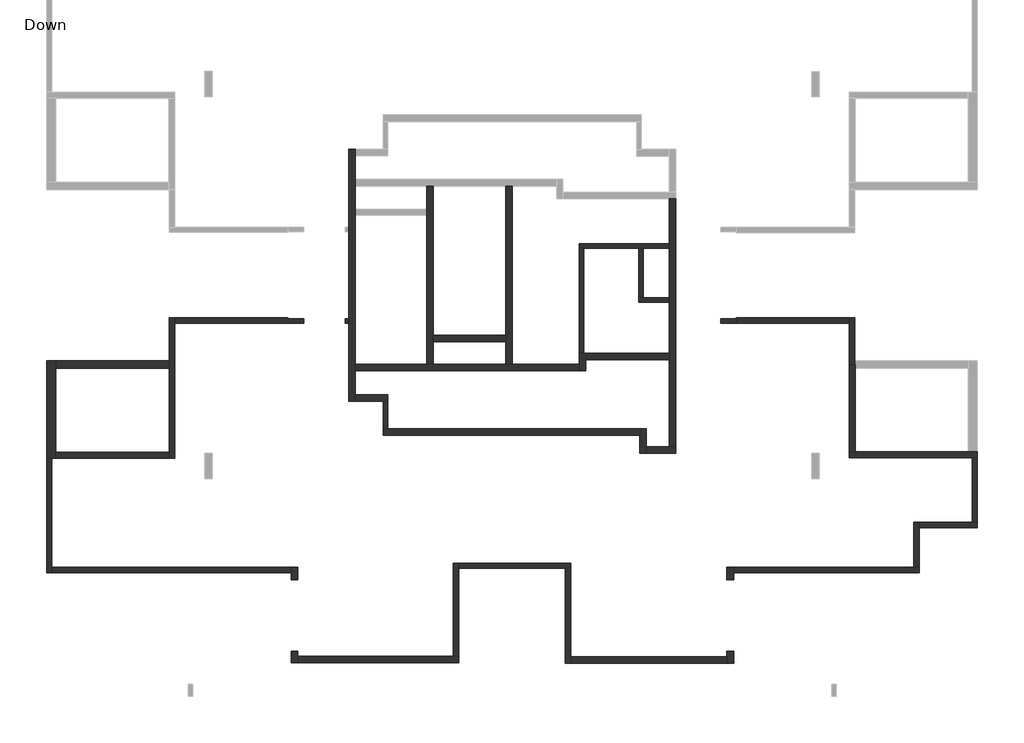
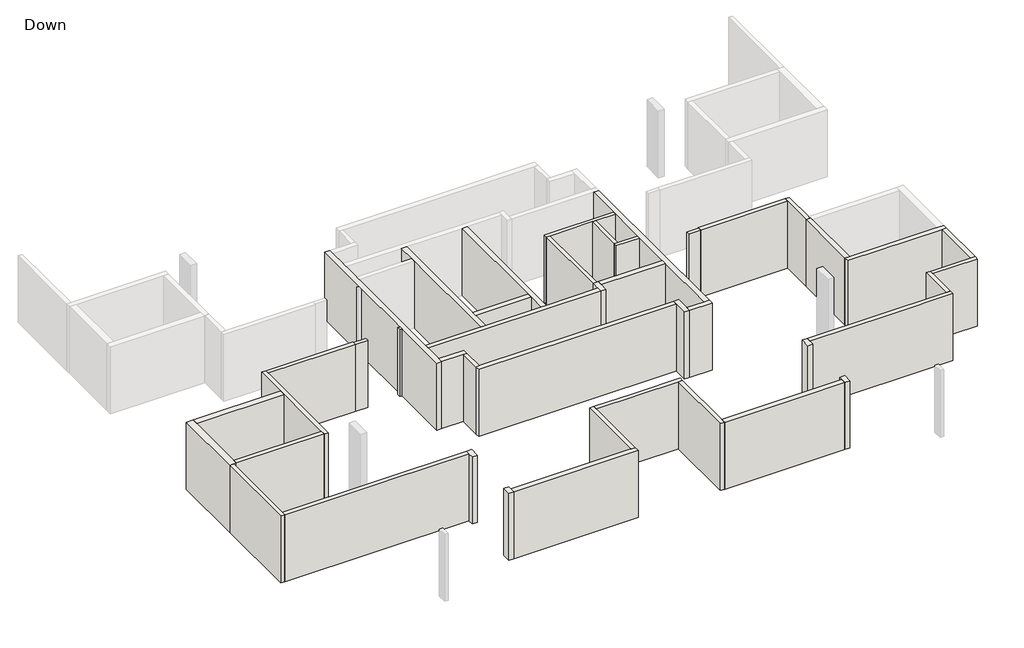
# One storey, part 1 of 2: 44 walls.
"""IFC4 building model written with IfcOpenShell, lengths in millimetres."""

from ifc_helpers import new_model, si_unit, origin, origin_with_axes, place, context, project, spatial, polyline, outline, extrude, faceted_brep, element, save

model = new_model("IFC4")

# Units and contexts
model_context = context("Model", 3, world=origin())
ifc_project = project(units=[si_unit("LENGTHUNIT", "METRE", prefix="MILLI")], contexts=[model_context])

# Site, building, storey
site = spatial("IfcSite", under=ifc_project)
building = spatial("IfcBuilding", under=site)
storey = spatial("IfcBuildingStorey", under=building, Name="Down", Elevation=0.0)

# Walls
placement = place(None, origin())
element("IfcWall", 1, ObjectType="15", at=placement, inside=storey, context=model_context, shape_type="Brep", body=[
    faceted_brep([(3307.48852, -2656.5516458, 0.0), (3822.84243, -2656.5516458, 0.0), (3822.84243, -2656.5516458, 3070.0), (3307.48852, -2656.5516458, 3070.0), (3307.48852, -2506.5516458, 0.0), (3307.48852, -2506.5516458, 3070.0), (3822.84243, -2506.5516458, 3070.0), (3822.84243, -2506.5516458, 2920.0), (3822.84243, -2506.5516458, 0.0), (3822.84243, -2656.2878227, 0.0), (3822.84243, -2656.2878227, 3070.0)], [[[0, 1, 2, 3]], [[4, 5, 6, 7, 8]], [[1, 0, 4, 8, 9]], [[2, 1, 9, 8, 7, 6, 10]], [[3, 2, 10, 6, 5]], [[0, 3, 5, 4]]]),
])
element("IfcWall", 2, ObjectType="15", at=placement, inside=storey, context=model_context, shape_type="Brep", body=[
    faceted_brep([(-11137.3486135, -2656.5516458, 0.0), (-10610.0280472, -2656.5516458, 0.0), (-10610.0280472, -2656.5516458, 2870.0), (-10610.0280472, -2656.5516458, 3070.0), (-11137.3486135, -2656.5516458, 3070.0), (-11137.3486135, -2656.5516458, 2870.0), (-11137.3486135, -2506.5516458, 0.0), (-11137.3486135, -2506.5516458, 2920.0), (-11137.3486135, -2506.5516458, 3070.0), (-10610.0280472, -2506.5516458, 3070.0), (-10610.0280472, -2506.5516458, 0.0), (-11137.3486135, -2656.2878227, 0.0), (-10610.0280472, -2655.7878227, 3070.0), (-11137.3486135, -2656.2878227, 3070.0)], [[[0, 1, 2, 3, 4, 5]], [[6, 7, 8, 9, 10]], [[1, 0, 11, 6, 10]], [[3, 2, 1, 10, 9, 12]], [[4, 3, 12, 9, 8, 13]], [[0, 5, 4, 13, 8, 7, 6, 11]]]),
])
element("IfcWall", 3, ObjectType="15", at=placement, inside=storey, context=model_context, shape_type="Brep", body=[
    faceted_brep([(-1415.2062248, -154.9895964, 0.0), (-1265.2062248, -154.9895964, 0.0), (579.9772808, -154.9895964, 0.0), (729.9772808, -154.9895964, 0.0), (1589.3005209, -154.9895964, 0.0), (1589.3005209, -154.9895964, 3070.0), (729.9772808, -154.9895964, 3070.0), (579.9772808, -154.9895964, 3070.0), (-1265.2062248, -154.9895964, 3070.0), (-1415.2062248, -154.9895964, 3070.0), (-1415.2062248, -4.9895964, 0.0), (-1415.2062248, -4.9895964, 2870.0), (-1415.2062248, -4.9895964, 3070.0), (1589.3005209, -4.9895964, 3070.0), (1589.3005209, -4.9895964, 2870.0), (1589.3005209, -4.9895964, 0.0)], [[[0, 1, 2, 3, 4, 5, 6, 7, 8, 9]], [[10, 11, 12, 13, 14, 15]], [[4, 3, 2, 1, 0, 10, 15]], [[9, 8, 7, 6, 5, 13, 12]], [[5, 4, 15, 14, 13]], [[0, 9, 12, 11, 10]]]),
])
element("IfcWall", 4, ObjectType="15", at=placement, inside=storey, context=model_context, shape_type="Brep", body=[
    faceted_brep([(1589.3005209, -1810.18983, 0.0), (729.9772808, -1810.18983, 0.0), (579.9772808, -1810.18983, 0.0), (579.9772808, -1810.18983, 3070.0), (729.9772808, -1810.18983, 3070.0), (1589.3005209, -1810.18983, 3070.0), (1589.3005209, -1960.18983, 0.0), (1589.3005209, -1960.18983, 3070.0), (579.9772808, -1960.18983, 3070.0), (579.9772808, -1960.18983, 0.0)], [[[0, 1, 2, 3, 4, 5]], [[6, 7, 8, 9]], [[2, 1, 0, 6, 9]], [[5, 4, 3, 8, 7]], [[0, 5, 7, 6]], [[3, 2, 9, 8]]]),
])
element("IfcWall", 5, ObjectType="15", at=placement, inside=storey, context=model_context, shape_type="SweptSolid", body=[
    extrude(outline(polyline([(579.9772808, -1810.18983), (579.9772808, -154.9895964), (729.9772808, -154.9895964), (729.9772808, -1810.18983), (579.9772808, -1810.18983)])), origin_with_axes(), (0.0, 0.0, 1.0), 3070.0),
])
element("IfcWall", 6, ObjectType="15", at=placement, inside=storey, context=model_context, shape_type="SweptSolid", body=[
    extrude(outline(polyline([(-1415.2062248, -3664.0679171), (-1415.2062248, -154.9895964), (-1265.2062248, -154.9895964), (-1265.2062248, -3664.0679171), (-1415.2062248, -3664.0679171)])), origin_with_axes(), (0.0, 0.0, 1.0), 3070.0),
])
element("IfcWall", 7, ObjectType="15", at=placement, inside=storey, context=model_context, shape_type="Brep", body=[
    faceted_brep([(-7960.7109614, -5263.3286489, 0.0), (-7960.7109614, -6190.6239212, 0.0), (-7960.7109614, -6190.6239212, 3070.0), (-7960.7109614, -5263.3286489, 3070.0), (-7960.7109614, -5263.3286489, 2870.0), (-7810.7109614, -5263.3286489, 0.0), (-7810.7109614, -5263.3286489, 3070.0), (-7810.7109614, -6190.6239212, 3070.0), (-7810.7109614, -6190.6239212, 2870.0), (-7810.7109614, -6190.6239212, 0.0)], [[[0, 1, 2, 3, 4]], [[5, 6, 7, 8, 9]], [[1, 0, 5, 9]], [[3, 2, 7, 6]], [[0, 4, 3, 6, 5]], [[2, 1, 9, 8, 7]]]),
])
element("IfcWall", 8, ObjectType="15", at=placement, inside=storey, context=model_context, shape_type="Brep", body=[
    faceted_brep([(-9219.5481077, -2656.5516458, 0.0), (-9111.0923752, -2656.5516458, 0.0), (-9111.0923752, -2656.5516458, 2870.0), (-9111.0923752, -2656.5516458, 3070.0), (-9219.5481077, -2656.5516458, 3070.0), (-9219.5481077, -2656.5516458, 2870.0), (-9219.5481077, -2506.5516458, 0.0), (-9219.5481077, -2506.5516458, 3070.0), (-9111.0923752, -2506.5516458, 3070.0), (-9111.0923752, -2506.5516458, 2920.0), (-9111.0923752, -2506.5516458, 0.0), (-9219.5481077, -2655.7878227, 3070.0)], [[[0, 1, 2, 3, 4, 5]], [[6, 7, 8, 9, 10]], [[1, 0, 6, 10]], [[4, 3, 8, 7, 11]], [[0, 5, 4, 11, 7, 6]], [[3, 2, 1, 10, 9, 8]]]),
])
element("IfcWall", 9, ObjectType="18", at=placement, inside=storey, context=model_context, shape_type="Brep", body=[
    faceted_brep([(-15093.3730612, -2476.2878227, 0.0), (-15093.3730612, -3916.1341463, 0.0), (-15093.3730612, -4166.1341463, 0.0), (-15093.3730612, -6966.8226087, 0.0), (-15093.3730612, -7166.8226087, 0.0), (-15093.3730612, -7166.8226087, 3070.0), (-15093.3730612, -6966.8226087, 3070.0), (-15093.3730612, -4166.1341463, 3070.0), (-15093.3730612, -3916.1341463, 3070.0), (-15093.3730612, -2476.2878227, 3070.0), (-14913.3730612, -2476.2878227, 0.0), (-14913.3730612, -2476.2878227, 3070.0), (-14913.3730612, -2656.2878227, 3070.0), (-14913.3730612, -7166.8226087, 3070.0), (-14913.3730612, -7166.8226087, 2870.0), (-14913.3730612, -7166.8226087, 0.0), (-14913.3730612, -2656.2878227, 0.0)], [[[0, 1, 2, 3, 4, 5, 6, 7, 8, 9]], [[10, 11, 12, 13, 14, 15, 16]], [[4, 3, 2, 1, 0, 10, 16, 15]], [[9, 8, 7, 6, 5, 13, 12, 11]], [[5, 4, 15, 14, 13]], [[0, 9, 11, 10]]]),
])
element("IfcWall", 10, ObjectType="18", at=placement, inside=storey, context=model_context, shape_type="Brep", body=[
    faceted_brep([(-19192.7470995, -7166.8226087, 0.0), (-19192.7470995, -10993.4504981, 0.0), (-19192.7470995, -10993.4504981, 3070.0), (-19192.7470995, -7166.8226087, 3070.0), (-19012.7470995, -7166.8226087, 0.0), (-19012.7470995, -7166.8226087, 2870.0), (-19012.7470995, -7166.8226087, 3070.0), (-19012.7470995, -10813.4504981, 3070.0), (-19012.7470995, -10993.4504981, 3070.0), (-19012.7470995, -10993.4504981, 0.0), (-19012.7470995, -10813.4504981, 0.0)], [[[0, 1, 2, 3]], [[4, 5, 6, 7, 8, 9, 10]], [[1, 0, 4, 10, 9]], [[3, 2, 8, 7, 6]], [[0, 3, 6, 5, 4]], [[2, 1, 9, 8]]]),
])
element("IfcWall", 11, ObjectType="18", at=placement, inside=storey, context=model_context, shape_type="Brep", body=[
    faceted_brep([(-19012.7470995, -10993.4504981, 0.0), (-11029.6404044, -10993.4504981, 0.0), (-11029.6404044, -10993.4504981, 2870.0), (-11029.6404044, -10993.4504981, 3070.0), (-14463.9862657, -10993.4504981, 3070.0), (-19012.7470995, -10993.4504981, 3070.0), (-19012.7470995, -10813.4504981, 0.0), (-19012.7470995, -10813.4504981, 2870.0), (-19012.7470995, -10813.4504981, 3070.0), (-11029.6404044, -10813.4504981, 3070.0), (-11029.6404044, -10813.4504981, 0.0)], [[[0, 1, 2, 3, 4, 5]], [[6, 7, 8, 9, 10]], [[1, 0, 6, 10]], [[5, 4, 3, 9, 8]], [[0, 5, 8, 7, 6]], [[3, 2, 1, 10, 9]]]),
])
element("IfcWall", 12, ObjectType="18", at=placement, inside=storey, context=model_context, shape_type="Brep", body=[
    faceted_brep([(-5611.3302453, -10669.5773003, 0.0), (-5611.3302453, -13772.0681688, 0.0), (-5611.3302453, -13772.0681688, 2870.0), (-5611.3302453, -13772.0681688, 3070.0), (-5611.3302453, -10669.5773003, 3070.0), (-5611.3302453, -10669.5773003, 2870.0), (-5431.3302453, -10669.5773003, 0.0), (-5431.3302453, -10669.5773003, 3070.0), (-5431.3302453, -10849.5773003, 3070.0), (-5431.3302453, -13772.0681688, 3070.0), (-5431.3302453, -13772.0681688, 0.0), (-5431.3302453, -10849.5773003, 0.0)], [[[0, 1, 2, 3, 4, 5]], [[6, 7, 8, 9, 10, 11]], [[1, 0, 6, 11, 10]], [[4, 3, 9, 8, 7]], [[3, 2, 1, 10, 9]], [[0, 5, 4, 7, 6]]]),
])
element("IfcWall", 13, ObjectType="18", at=placement, inside=storey, context=model_context, shape_type="Brep", body=[
    faceted_brep([(-5431.3302453, -10849.5773003, 0.0), (-1871.2080852, -10849.5773003, 0.0), (-1691.2080852, -10849.5773003, 0.0), (-1691.2080852, -10849.5773003, 3070.0), (-1871.2080852, -10849.5773003, 3070.0), (-5431.3302453, -10849.5773003, 3070.0), (-5431.3302453, -10669.5773003, 0.0), (-5431.3302453, -10669.5773003, 3070.0), (-3748.3678079, -10669.5773003, 3070.0), (-3553.3678079, -10669.5773003, 3070.0), (-1691.2080852, -10669.5773003, 3070.0), (-1691.2080852, -10669.5773003, 2870.0), (-1691.2080852, -10669.5773003, 0.0)], [[[0, 1, 2, 3, 4, 5]], [[6, 7, 8, 9, 10, 11, 12]], [[2, 1, 0, 6, 12]], [[5, 4, 3, 10, 9, 8, 7]], [[0, 5, 7, 6]], [[3, 2, 12, 11, 10]]]),
])
element("IfcWall", 14, ObjectType="18", at=placement, inside=storey, context=model_context, shape_type="Brep", body=[
    faceted_brep([(-1871.2080852, -10849.5773003, 0.0), (-1871.2080852, -14009.5773003, 0.0), (-1871.2080852, -14009.5773003, 3070.0), (-1871.2080852, -10849.5773003, 3070.0), (-1691.2080852, -10849.5773003, 0.0), (-1691.2080852, -10849.5773003, 3070.0), (-1691.2080852, -13789.5773003, 3070.0), (-1691.2080852, -14009.5773003, 3070.0), (-1691.2080852, -14009.5773003, 0.0), (-1691.2080852, -13789.5773003, 0.0)], [[[0, 1, 2, 3]], [[4, 5, 6, 7, 8, 9]], [[1, 0, 4, 9, 8]], [[3, 2, 7, 6, 5]], [[0, 3, 5, 4]], [[2, 1, 8, 7]]]),
])
element("IfcWall", 15, ObjectType="18", at=placement, inside=storey, context=model_context, shape_type="Brep", body=[
    faceted_brep([(9937.2529005, -10813.4467583, 0.0), (9757.2529005, -10813.4467583, 0.0), (3739.0676082, -10813.4467583, 0.0), (3739.0676082, -10813.4467583, 3070.0), (9757.2529005, -10813.4467583, 3070.0), (9937.2529005, -10813.4467583, 3070.0), (9937.2529005, -10993.4467583, 0.0), (9937.2529005, -10993.4467583, 3070.0), (7161.4479352, -10993.4467583, 3070.0), (3739.0676082, -10993.4467583, 3070.0), (3739.0676082, -10993.4467583, 2870.0), (3739.0676082, -10993.4467583, 0.0)], [[[0, 1, 2, 3, 4, 5]], [[6, 7, 8, 9, 10, 11]], [[2, 1, 0, 6, 11]], [[5, 4, 3, 9, 8, 7]], [[0, 5, 7, 6]], [[3, 2, 11, 10, 9]]]),
])
element("IfcWall", 16, ObjectType="18", at=placement, inside=storey, context=model_context, shape_type="Brep", body=[
    faceted_brep([(9757.2529005, -9313.7627402, 0.0), (9757.2529005, -10813.4467583, 0.0), (9757.2529005, -10813.4467583, 2870.0), (9757.2529005, -10813.4467583, 3070.0), (9757.2529005, -9313.7627402, 3070.0), (9757.2529005, -9313.7627402, 2870.0), (9937.2529005, -9313.7627402, 0.0), (9937.2529005, -9313.7627402, 3070.0), (9937.2529005, -9493.7627402, 3070.0), (9937.2529005, -10813.4467583, 3070.0), (9937.2529005, -10813.4467583, 0.0), (9937.2529005, -9493.7627402, 0.0)], [[[0, 1, 2, 3, 4, 5]], [[6, 7, 8, 9, 10, 11]], [[1, 0, 6, 11, 10]], [[4, 3, 9, 8, 7]], [[3, 2, 1, 10, 9]], [[0, 5, 4, 7, 6]]]),
])
element("IfcWall", 17, ObjectType="18", at=placement, inside=storey, context=model_context, shape_type="Brep", body=[
    faceted_brep([(9937.2529005, -9493.7627402, 0.0), (11878.5007748, -9493.7627402, 0.0), (11878.5007748, -9493.7627402, 3070.0), (9937.2529005, -9493.7627402, 3070.0), (9937.2529005, -9313.7627402, 0.0), (9937.2529005, -9313.7627402, 3070.0), (11698.5007748, -9313.7627402, 3070.0), (11878.5007748, -9313.7627402, 3070.0), (11878.5007748, -9313.7627402, 0.0), (11698.5007748, -9313.7627402, 0.0)], [[[0, 1, 2, 3]], [[4, 5, 6, 7, 8, 9]], [[1, 0, 4, 9, 8]], [[3, 2, 7, 6, 5]], [[0, 3, 5, 4]], [[2, 1, 8, 7]]]),
])
element("IfcWall", 18, ObjectType="18", at=placement, inside=storey, context=model_context, shape_type="Brep", body=[
    faceted_brep([(11878.5007748, -9313.7627402, 0.0), (11878.5007748, -7153.7627402, 0.0), (11878.5007748, -7153.7627402, 3070.0), (11878.5007748, -9313.7627402, 3070.0), (11698.5007748, -9313.7627402, 0.0), (11698.5007748, -9313.7627402, 2870.0), (11698.5007748, -9313.7627402, 3070.0), (11698.5007748, -7153.7627402, 3070.0), (11698.5007748, -7153.7627402, 2870.0), (11698.5007748, -7153.7627402, 0.0)], [[[0, 1, 2, 3]], [[4, 5, 6, 7, 8, 9]], [[1, 0, 4, 9]], [[3, 2, 7, 6]], [[0, 3, 6, 5, 4]], [[2, 1, 9, 8, 7]]]),
])
element("IfcWall", 19, ObjectType="18", at=placement, inside=storey, context=model_context, shape_type="Brep", body=[
    faceted_brep([(7780.4432059, -4041.1341463, 0.0), (7780.4432059, -3916.1341463, 0.0), (7780.4432059, -2476.2878227, 0.0), (7780.4432059, -2476.2878227, 3070.0), (7780.4432059, -3916.1341463, 3070.0), (7780.4432059, -4041.1341463, 3070.0), (7600.4432059, -4041.1341463, 0.0), (7600.4432059, -4041.1341463, 3070.0), (7600.4432059, -2656.5516458, 3070.0), (7600.4432059, -2656.2878227, 3070.0), (7600.4432059, -2476.2878227, 3070.0), (7600.4432059, -2476.2878227, 0.0), (7600.4432059, -2656.2878227, 0.0)], [[[0, 1, 2, 3, 4, 5]], [[6, 7, 8, 9, 10, 11, 12]], [[2, 1, 0, 6, 12, 11]], [[5, 4, 3, 10, 9, 8, 7]], [[0, 5, 7, 6]], [[3, 2, 11, 10]]]),
])
element("IfcWall", 20, ObjectType="18", at=placement, inside=storey, context=model_context, shape_type="Brep", body=[
    faceted_brep([(7600.4432059, -2476.2878227, 0.0), (3822.84243, -2476.2878227, 0.0), (3822.84243, -2476.2878227, 3070.0), (7600.4432059, -2476.2878227, 3070.0), (7600.4432059, -2656.2878227, 0.0), (7600.4432059, -2656.2878227, 3070.0), (3822.84243, -2656.2878227, 3070.0), (3822.84243, -2656.2878227, 0.0), (3822.84243, -2506.5516458, 0.0), (3822.84243, -2506.5516458, 3070.0)], [[[0, 1, 2, 3]], [[4, 5, 6, 7]], [[1, 0, 4, 7, 8]], [[2, 1, 8, 7, 6, 9]], [[3, 2, 9, 6, 5]], [[0, 3, 5, 4]]]),
])
element("IfcWall", 21, ObjectType="18", at=placement, inside=storey, context=model_context, shape_type="Brep", body=[
    faceted_brep([(-14913.3730612, -2656.2878227, 0.0), (-11137.3486135, -2656.2878227, 0.0), (-11137.3486135, -2656.2878227, 2870.0), (-11137.3486135, -2656.2878227, 3070.0), (-14913.3730612, -2656.2878227, 3070.0), (-14913.3730612, -2656.2878227, 2870.0), (-14913.3730612, -2476.2878227, 0.0), (-14913.3730612, -2476.2878227, 3070.0), (-11137.3486135, -2476.2878227, 3070.0), (-11137.3486135, -2476.2878227, 0.0), (-11137.3486135, -2506.5516458, 0.0), (-11137.3486135, -2506.5516458, 3070.0)], [[[0, 1, 2, 3, 4, 5]], [[6, 7, 8, 9]], [[1, 0, 6, 9, 10]], [[3, 2, 1, 10, 9, 8, 11]], [[4, 3, 11, 8, 7]], [[0, 5, 4, 7, 6]]]),
])
element("IfcWall", 22, ObjectType="20", at=placement, inside=storey, context=model_context, shape_type="Brep", body=[
    faceted_brep([(-15093.3730612, -6966.8226087, 0.0), (-18893.0716357, -6966.8226087, 0.0), (-18893.0716357, -6966.8226087, 2870.0), (-18893.0716357, -6966.8226087, 3070.0), (-15093.3730612, -6966.8226087, 3070.0), (-15093.3730612, -6966.8226087, 2870.0), (-15093.3730612, -7166.8226087, 0.0), (-15093.3730612, -7166.8226087, 3070.0), (-18893.0716357, -7166.8226087, 3070.0), (-18893.0716357, -7166.8226087, 0.0)], [[[0, 1, 2, 3, 4, 5]], [[6, 7, 8, 9]], [[1, 0, 6, 9]], [[4, 3, 8, 7]], [[3, 2, 1, 9, 8]], [[0, 5, 4, 7, 6]]]),
])
element("IfcWall", 23, ObjectType="20", at=placement, inside=storey, context=model_context, shape_type="Brep", body=[
    faceted_brep([(11879.3119283, -6953.7627402, 0.0), (11579.3119283, -6953.7627402, 0.0), (7800.4432059, -6953.7627402, 0.0), (7600.4432059, -6953.7627402, 0.0), (7600.4432059, -6953.7627402, 3070.0), (7800.4432059, -6953.7627402, 3070.0), (11579.3119283, -6953.7627402, 3070.0), (11879.3119283, -6953.7627402, 3070.0), (11879.3119283, -7153.7627402, 0.0), (11879.3119283, -7153.7627402, 3070.0), (11878.5007748, -7153.7627402, 3070.0), (11698.5007748, -7153.7627402, 3070.0), (7600.4432059, -7153.7627402, 3070.0), (7600.4432059, -7153.7627402, 2870.0), (7600.4432059, -7153.7627402, 0.0), (11698.5007748, -7153.7627402, 0.0), (11878.5007748, -7153.7627402, 0.0)], [[[0, 1, 2, 3, 4, 5, 6, 7]], [[8, 9, 10, 11, 12, 13, 14, 15, 16]], [[3, 2, 1, 0, 8, 16, 15, 14]], [[7, 6, 5, 4, 12, 11, 10, 9]], [[0, 7, 9, 8]], [[4, 3, 14, 13, 12]]]),
])
element("IfcWall", 24, ObjectType="20", at=placement, inside=storey, context=model_context, shape_type="Brep", body=[
    faceted_brep([(7800.4432059, -6953.7627402, 0.0), (7800.4432059, -4166.1341463, 0.0), (7800.4432059, -4041.1341463, 0.0), (7800.4432059, -4041.1341463, 3070.0), (7800.4432059, -4166.1341463, 3070.0), (7800.4432059, -6953.7627402, 3070.0), (7800.4432059, -6953.7627402, 2870.0), (7600.4432059, -6953.7627402, 0.0), (7600.4432059, -6953.7627402, 3070.0), (7600.4432059, -4041.1341463, 3070.0), (7600.4432059, -4041.1341463, 0.0), (7780.4432059, -4041.1341463, 0.0), (7780.4432059, -4041.1341463, 3070.0)], [[[0, 1, 2, 3, 4, 5, 6]], [[7, 8, 9, 10]], [[2, 1, 0, 7, 10, 11]], [[3, 2, 11, 10, 9, 12]], [[5, 4, 3, 12, 9, 8]], [[0, 6, 5, 8, 7]]]),
])
element("IfcWall", 25, ObjectType="22", at=placement, inside=storey, context=model_context, shape_type="Brep", body=[
    faceted_brep([(-10809.6404044, -13992.0681688, 0.0), (-5431.0686661, -13992.0681688, 0.0), (-5431.0686661, -13992.0681688, 3070.0), (-10809.6404044, -13992.0681688, 3070.0), (-10809.6404044, -13772.0681688, 0.0), (-10809.6404044, -13772.0681688, 2870.0), (-10809.6404044, -13772.0681688, 3070.0), (-5611.3302453, -13772.0681688, 3070.0), (-5431.3302453, -13772.0681688, 3070.0), (-5431.0686661, -13772.0681688, 3070.0), (-5431.0686661, -13772.0681688, 0.0), (-5431.3302453, -13772.0681688, 0.0), (-5611.3302453, -13772.0681688, 0.0)], [[[0, 1, 2, 3]], [[4, 5, 6, 7, 8, 9, 10, 11, 12]], [[1, 0, 4, 12, 11, 10]], [[2, 1, 10, 9]], [[3, 2, 9, 8, 7, 6]], [[0, 3, 6, 5, 4]]]),
])
element("IfcWall", 26, ObjectType="22", at=placement, inside=storey, context=model_context, shape_type="Brep", body=[
    faceted_brep([(3519.0676082, -13789.5773003, 0.0), (-1691.2080852, -13789.5773003, 0.0), (-1691.2080852, -13789.5773003, 2870.0), (-1691.2080852, -13789.5773003, 3070.0), (3519.0676082, -13789.5773003, 3070.0), (3519.0676082, -13789.5773003, 2870.0), (3519.0676082, -14009.5773003, 0.0), (3519.0676082, -14009.5773003, 3070.0), (-1691.2080852, -14009.5773003, 3070.0), (-1691.2080852, -14009.5773003, 0.0)], [[[0, 1, 2, 3, 4, 5]], [[6, 7, 8, 9]], [[1, 0, 6, 9]], [[4, 3, 8, 7]], [[3, 2, 1, 9, 8]], [[0, 5, 4, 7, 6]]]),
])
element("IfcWall", 27, ObjectType="22", at=placement, inside=storey, context=model_context, shape_type="Brep", body=[
    faceted_brep([(-8891.0923752, -5263.3286489, 0.0), (-8891.0923752, -5043.3286489, 0.0), (-8891.0923752, -4251.9774411, 0.0), (-8891.0923752, -4031.9774411, 0.0), (-8891.0923752, 942.6898033, 0.0), (-8891.0923752, 1142.6898033, 0.0), (-8891.0923752, 1914.3048342, 0.0), (-8891.0923752, 2134.3048342, 0.0), (-8891.0923752, 2921.8256682, 0.0), (-8891.0923752, 3141.8256682, 0.0), (-8891.0923752, 3141.8256682, 3070.0), (-8891.0923752, 2921.8256682, 3070.0), (-8891.0923752, 2134.3048342, 3070.0), (-8891.0923752, 1914.3048342, 3070.0), (-8891.0923752, 1142.6898033, 3070.0), (-8891.0923752, 942.6898033, 3070.0), (-8891.0923752, -4031.9774411, 3070.0), (-8891.0923752, -4251.9774411, 3070.0), (-8891.0923752, -5043.3286489, 3070.0), (-8891.0923752, -5263.3286489, 3070.0), (-9111.0923752, -5263.3286489, 0.0), (-9111.0923752, -5263.3286489, 2870.0), (-9111.0923752, -5263.3286489, 3070.0), (-9111.0923752, -2656.5516458, 3070.0), (-9111.0923752, -2506.5516458, 3070.0), (-9111.0923752, 396.2654793, 3070.0), (-9111.0923752, 546.2654793, 3070.0), (-9111.0923752, 3141.8256682, 3070.0), (-9111.0923752, 3141.8256682, 2870.0), (-9111.0923752, 3141.8256682, 0.0), (-9111.0923752, 546.2654793, 0.0), (-9111.0923752, 396.2654793, 0.0), (-9111.0923752, -2506.5516458, 0.0), (-9111.0923752, -2656.5516458, 0.0)], [[[0, 1, 2, 3, 4, 5, 6, 7, 8, 9, 10, 11, 12, 13, 14, 15, 16, 17, 18, 19]], [[20, 21, 22, 23, 24, 25, 26, 27, 28, 29, 30, 31, 32, 33]], [[9, 8, 7, 6, 5, 4, 3, 2, 1, 0, 20, 33, 32, 31, 30, 29]], [[19, 18, 17, 16, 15, 14, 13, 12, 11, 10, 27, 26, 25, 24, 23, 22]], [[10, 9, 29, 28, 27]], [[0, 19, 22, 21, 20]]]),
])
element("IfcWall", 28, ObjectType="22", at=placement, inside=storey, context=model_context, shape_type="Brep", body=[
    faceted_brep([(-7810.7109614, -5043.3286489, 0.0), (-8891.0923752, -5043.3286489, 0.0), (-8891.0923752, -5043.3286489, 2870.0), (-8891.0923752, -5043.3286489, 3070.0), (-7810.7109614, -5043.3286489, 3070.0), (-7810.7109614, -5043.3286489, 2870.0), (-7810.7109614, -5263.3286489, 0.0), (-7810.7109614, -5263.3286489, 3070.0), (-7960.7109614, -5263.3286489, 3070.0), (-8891.0923752, -5263.3286489, 3070.0), (-8891.0923752, -5263.3286489, 0.0), (-7960.7109614, -5263.3286489, 0.0)], [[[0, 1, 2, 3, 4, 5]], [[6, 7, 8, 9, 10, 11]], [[1, 0, 6, 11, 10]], [[4, 3, 9, 8, 7]], [[3, 2, 1, 10, 9]], [[0, 5, 4, 7, 6]]]),
])
element("IfcWall", 29, ObjectType="22", at=placement, inside=storey, context=model_context, shape_type="Brep", body=[
    faceted_brep([(-7960.7109614, -6410.6239212, 0.0), (610.3012935, -6410.6239212, 0.0), (610.3012935, -6410.6239212, 2870.0), (610.3012935, -6410.6239212, 3070.0), (-3553.3678079, -6410.6239212, 3070.0), (-3748.3678079, -6410.6239212, 3070.0), (-7960.7109614, -6410.6239212, 3070.0), (-7960.7109614, -6410.6239212, 2870.0), (-7960.7109614, -6190.6239212, 0.0), (-7960.7109614, -6190.6239212, 3070.0), (-7810.7109614, -6190.6239212, 3070.0), (610.3012935, -6190.6239212, 3070.0), (610.3012935, -6190.6239212, 0.0), (-7810.7109614, -6190.6239212, 0.0)], [[[0, 1, 2, 3, 4, 5, 6, 7]], [[8, 9, 10, 11, 12, 13]], [[1, 0, 8, 13, 12]], [[6, 5, 4, 3, 11, 10, 9]], [[0, 7, 6, 9, 8]], [[3, 2, 1, 12, 11]]]),
])
element("IfcWall", 30, ObjectType="22", at=placement, inside=storey, context=model_context, shape_type="Brep", body=[
    faceted_brep([(1809.3005209, -6790.4989795, 0.0), (1589.3005209, -6790.4989795, 0.0), (830.3012935, -6790.4989795, 0.0), (830.3012935, -6790.4989795, 2870.0), (830.3012935, -6790.4989795, 3070.0), (1589.3005209, -6790.4989795, 3070.0), (1809.3005209, -6790.4989795, 3070.0), (1809.3005209, -7010.4989795, 0.0), (1809.3005209, -7010.4989795, 2870.0), (1809.3005209, -7010.4989795, 3070.0), (830.3012935, -7010.4989795, 3070.0), (830.3012935, -7010.4989795, 0.0)], [[[0, 1, 2, 3, 4, 5, 6]], [[7, 8, 9, 10, 11]], [[2, 1, 0, 7, 11]], [[6, 5, 4, 10, 9]], [[4, 3, 2, 11, 10]], [[0, 6, 9, 8, 7]]]),
])
element("IfcWall", 31, ObjectType="22", at=placement, inside=storey, context=model_context, shape_type="Brep", body=[
    faceted_brep([(1809.3005209, -6790.4989795, 0.0), (1809.3005209, 1493.9448789, 0.0), (1809.3005209, 1493.9448789, 3070.0), (1809.3005209, 540.6860076, 3070.0), (1809.3005209, 390.6860076, 3070.0), (1809.3005209, -2506.5516458, 3070.0), (1809.3005209, -2656.5516458, 3070.0), (1809.3005209, -6790.4989795, 3070.0), (1589.3005209, -6790.4989795, 0.0), (1589.3005209, -6790.4989795, 2870.0), (1589.3005209, -6790.4989795, 3070.0), (1589.3005209, -3884.0679171, 3070.0), (1589.3005209, -3664.0679171, 3070.0), (1589.3005209, -1960.18983, 3070.0), (1589.3005209, -1810.18983, 3070.0), (1589.3005209, -154.9895964, 3070.0), (1589.3005209, -4.9895964, 3070.0), (1589.3005209, 1493.9448789, 3070.0), (1589.3005209, 1493.9448789, 2870.0), (1589.3005209, 1493.9448789, 0.0), (1589.3005209, -4.9895964, 0.0), (1589.3005209, -154.9895964, 0.0), (1589.3005209, -1810.18983, 0.0), (1589.3005209, -1960.18983, 0.0), (1589.3005209, -3664.0679171, 0.0), (1589.3005209, -3884.0679171, 0.0)], [[[0, 1, 2, 3, 4, 5, 6, 7]], [[8, 9, 10, 11, 12, 13, 14, 15, 16, 17, 18, 19, 20, 21, 22, 23, 24, 25]], [[1, 0, 8, 25, 24, 23, 22, 21, 20, 19]], [[7, 6, 5, 4, 3, 2, 17, 16, 15, 14, 13, 12, 11, 10]], [[2, 1, 19, 18, 17]], [[0, 7, 10, 9, 8]]]),
])
element("IfcWall", 32, ObjectType="22", at=placement, inside=storey, context=model_context, shape_type="Brep", body=[
    faceted_brep([(-1415.2062248, -4031.9774411, 0.0), (-3653.0437953, -4031.9774411, 0.0), (-3873.0437953, -4031.9774411, 0.0), (-6278.4263718, -4031.9774411, 0.0), (-6498.4263718, -4031.9774411, 0.0), (-8891.0923752, -4031.9774411, 0.0), (-8891.0923752, -4031.9774411, 2870.0), (-8891.0923752, -4031.9774411, 3070.0), (-6498.4263718, -4031.9774411, 3070.0), (-6278.4263718, -4031.9774411, 3070.0), (-3873.0437953, -4031.9774411, 3070.0), (-3653.0437953, -4031.9774411, 3070.0), (-1415.2062248, -4031.9774411, 3070.0), (-1415.2062248, -4031.9774411, 2870.0), (-1415.2062248, -4251.9774411, 0.0), (-1415.2062248, -4251.9774411, 3070.0), (-8891.0923752, -4251.9774411, 3070.0), (-8891.0923752, -4251.9774411, 2870.0), (-8891.0923752, -4251.9774411, 0.0)], [[[0, 1, 2, 3, 4, 5, 6, 7, 8, 9, 10, 11, 12, 13]], [[14, 15, 16, 17, 18]], [[5, 4, 3, 2, 1, 0, 14, 18]], [[12, 11, 10, 9, 8, 7, 16, 15]], [[7, 6, 5, 18, 17, 16]], [[0, 13, 12, 15, 14]]]),
])
element("IfcWall", 33, ObjectType="22", at=placement, inside=storey, context=model_context, shape_type="Brep", body=[
    faceted_brep([(-6278.4263718, -4031.9774411, 0.0), (-6278.4263718, -3284.1974214, 0.0), (-6278.4263718, -3064.1974214, 0.0), (-6278.4263718, 1914.3048342, 0.0), (-6278.4263718, 1914.3048342, 2870.0), (-6278.4263718, 1914.3048342, 3070.0), (-6278.4263718, -3064.1974214, 3070.0), (-6278.4263718, -3284.1974214, 3070.0), (-6278.4263718, -4031.9774411, 3070.0), (-6498.4263718, -4031.9774411, 0.0), (-6498.4263718, -4031.9774411, 2870.0), (-6498.4263718, -4031.9774411, 3070.0), (-6498.4263718, 942.6898033, 3070.0), (-6498.4263718, 1142.6898033, 3070.0), (-6498.4263718, 1914.3048342, 3070.0), (-6498.4263718, 1914.3048342, 0.0), (-6498.4263718, 1142.6898033, 0.0), (-6498.4263718, 942.6898033, 0.0)], [[[0, 1, 2, 3, 4, 5, 6, 7, 8]], [[9, 10, 11, 12, 13, 14, 15, 16, 17]], [[3, 2, 1, 0, 9, 17, 16, 15]], [[8, 7, 6, 5, 14, 13, 12, 11]], [[5, 4, 3, 15, 14]], [[0, 8, 11, 10, 9]]]),
])
element("IfcWall", 34, ObjectType="22", at=placement, inside=storey, context=model_context, shape_type="Brep", body=[
    faceted_brep([(-3653.0437953, -4031.9774411, 0.0), (-3653.0437953, 1914.3048342, 0.0), (-3653.0437953, 1914.3048342, 2870.0), (-3653.0437953, 1914.3048342, 3070.0), (-3653.0437953, -4031.9774411, 3070.0), (-3653.0437953, -4031.9774411, 2870.0), (-3873.0437953, -4031.9774411, 0.0), (-3873.0437953, -4031.9774411, 3070.0), (-3873.0437953, -3284.1974214, 3070.0), (-3873.0437953, -3064.1974214, 3070.0), (-3873.0437953, 1914.3048342, 3070.0), (-3873.0437953, 1914.3048342, 2870.0), (-3873.0437953, 1914.3048342, 0.0), (-3873.0437953, -3064.1974214, 0.0), (-3873.0437953, -3284.1974214, 0.0)], [[[0, 1, 2, 3, 4, 5]], [[6, 7, 8, 9, 10, 11, 12, 13, 14]], [[1, 0, 6, 14, 13, 12]], [[4, 3, 10, 9, 8, 7]], [[3, 2, 1, 12, 11, 10]], [[0, 5, 4, 7, 6]]]),
])
element("IfcWall", 35, ObjectType="22", at=placement, inside=storey, context=model_context, shape_type="Brep", body=[
    faceted_brep([(-3873.0437953, -3064.1974214, 0.0), (-6278.4263718, -3064.1974214, 0.0), (-6278.4263718, -3064.1974214, 2870.0), (-6278.4263718, -3064.1974214, 3070.0), (-3873.0437953, -3064.1974214, 3070.0), (-3873.0437953, -3064.1974214, 2870.0), (-3873.0437953, -3284.1974214, 0.0), (-3873.0437953, -3284.1974214, 3070.0), (-6278.4263718, -3284.1974214, 3070.0), (-6278.4263718, -3284.1974214, 0.0)], [[[0, 1, 2, 3, 4, 5]], [[6, 7, 8, 9]], [[1, 0, 6, 9]], [[4, 3, 8, 7]], [[0, 5, 4, 7, 6]], [[3, 2, 1, 9, 8]]]),
])
element("IfcWall", 36, ObjectType="22", at=placement, inside=storey, context=model_context, shape_type="Brep", body=[
    faceted_brep([(610.3012935, -6190.6239212, 0.0), (610.3012935, -6410.6239212, 0.0), (610.3012935, -7010.4989795, 0.0), (610.3012935, -7010.4989795, 2870.0), (610.3012935, -7010.4989795, 3070.0), (610.3012935, -6410.6239212, 3070.0), (610.3012935, -6190.6239212, 3070.0), (830.3012935, -6190.6239212, 0.0), (830.3012935, -6190.6239212, 2870.0), (830.3012935, -6190.6239212, 3070.0), (830.3012935, -6790.4989795, 3070.0), (830.3012935, -7010.4989795, 3070.0), (830.3012935, -7010.4989795, 0.0), (830.3012935, -6790.4989795, 0.0)], [[[0, 1, 2, 3, 4, 5, 6]], [[7, 8, 9, 10, 11, 12, 13]], [[2, 1, 0, 7, 13, 12]], [[6, 5, 4, 11, 10, 9]], [[0, 6, 9, 8, 7]], [[4, 3, 2, 12, 11]]]),
])
element("IfcWall", 37, ObjectType="22", at=placement, inside=storey, context=model_context, shape_type="Brep", body=[
    faceted_brep([(-1195.2062248, -3884.0679171, 0.0), (1589.3005209, -3884.0679171, 0.0), (1589.3005209, -3884.0679171, 2870.0), (1589.3005209, -3884.0679171, 3070.0), (-1195.2062248, -3884.0679171, 3070.0), (-1195.2062248, -3884.0679171, 2870.0), (-1195.2062248, -3664.0679171, 0.0), (-1195.2062248, -3664.0679171, 3070.0), (1589.3005209, -3664.0679171, 3070.0), (1589.3005209, -3664.0679171, 0.0)], [[[0, 1, 2, 3, 4, 5]], [[6, 7, 8, 9]], [[1, 0, 6, 9]], [[4, 3, 8, 7]], [[3, 2, 1, 9, 8]], [[0, 5, 4, 7, 6]]]),
])
element("IfcWall", 38, ObjectType="22", at=placement, inside=storey, context=model_context, shape_type="Brep", body=[
    faceted_brep([(-1415.2062248, -3664.0679171, 0.0), (-1415.2062248, -4031.9774411, 0.0), (-1415.2062248, -4251.9774411, 0.0), (-1415.2062248, -4251.9774411, 3070.0), (-1415.2062248, -4031.9774411, 3070.0), (-1415.2062248, -3664.0679171, 3070.0), (-1195.2062248, -3664.0679171, 0.0), (-1195.2062248, -3664.0679171, 3070.0), (-1195.2062248, -3884.0679171, 3070.0), (-1195.2062248, -4251.9774411, 3070.0), (-1195.2062248, -4251.9774411, 2870.0), (-1195.2062248, -4251.9774411, 0.0), (-1195.2062248, -3884.0679171, 0.0), (-1265.2062248, -3664.0679171, 0.0), (-1265.2062248, -3664.0679171, 3070.0)], [[[0, 1, 2, 3, 4, 5]], [[6, 7, 8, 9, 10, 11, 12]], [[2, 1, 0, 13, 6, 12, 11]], [[5, 4, 3, 9, 8, 7, 14]], [[3, 2, 11, 10, 9]], [[0, 5, 14, 7, 6, 13]]]),
])
element("IfcWall", 39, ObjectType="22", at=placement, inside=storey, context=model_context, shape_type="Brep", body=[
    faceted_brep([(-10809.6404044, -13992.0681688, 0.0), (-10809.6404044, -13772.0681688, 0.0), (-10809.6404044, -13620.3281962, 0.0), (-10809.6404044, -13620.3281962, 2420.0), (-10809.6404044, -13620.3281962, 3070.0), (-10809.6404044, -13772.0681688, 3070.0), (-10809.6404044, -13992.0681688, 3070.0), (-10809.6404044, -13992.0681688, 2870.0), (-11029.6404044, -13992.0681688, 0.0), (-11029.6404044, -13992.0681688, 2870.0), (-11029.6404044, -13992.0681688, 3070.0), (-11029.6404044, -13620.3281962, 3070.0), (-11029.6404044, -13620.3281962, 2420.0), (-11029.6404044, -13620.3281962, 0.0)], [[[0, 1, 2, 3, 4, 5, 6, 7]], [[8, 9, 10, 11, 12, 13]], [[2, 1, 0, 8, 13]], [[4, 3, 2, 13, 12, 11]], [[6, 5, 4, 11, 10]], [[0, 7, 6, 10, 9, 8]]]),
])
element("IfcWall", 40, ObjectType="22", at=placement, inside=storey, context=model_context, shape_type="Brep", body=[
    faceted_brep([(-11029.6404044, -10813.4504981, 0.0), (-11029.6404044, -10993.4504981, 0.0), (-11029.6404044, -11233.4504981, 0.0), (-11029.6404044, -11233.4504981, 2420.0), (-11029.6404044, -11233.4504981, 3070.0), (-11029.6404044, -10993.4504981, 3070.0), (-11029.6404044, -10813.4504981, 3070.0), (-10809.6404044, -10813.4504981, 0.0), (-10809.6404044, -10813.4504981, 2870.0), (-10809.6404044, -10813.4504981, 3070.0), (-10809.6404044, -11233.4504981, 3070.0), (-10809.6404044, -11233.4504981, 2420.0), (-10809.6404044, -11233.4504981, 0.0)], [[[0, 1, 2, 3, 4, 5, 6]], [[7, 8, 9, 10, 11, 12]], [[2, 1, 0, 7, 12]], [[4, 3, 2, 12, 11, 10]], [[6, 5, 4, 10, 9]], [[0, 6, 9, 8, 7]]]),
])
element("IfcWall", 41, ObjectType="22", at=placement, inside=storey, context=model_context, shape_type="Brep", body=[
    faceted_brep([(3739.0676082, -14009.5773003, 0.0), (3739.0676082, -13619.5773003, 0.0), (3739.0676082, -13619.5773003, 2420.0), (3739.0676082, -13619.5773003, 3070.0), (3739.0676082, -14009.5773003, 3070.0), (3739.0676082, -14009.5773003, 2870.0), (3519.0676082, -14009.5773003, 0.0), (3519.0676082, -14009.5773003, 2870.0), (3519.0676082, -14009.5773003, 3070.0), (3519.0676082, -13789.5773003, 3070.0), (3519.0676082, -13619.5773003, 3070.0), (3519.0676082, -13619.5773003, 2420.0), (3519.0676082, -13619.5773003, 0.0), (3519.0676082, -13789.5773003, 0.0)], [[[0, 1, 2, 3, 4, 5]], [[6, 7, 8, 9, 10, 11, 12, 13]], [[1, 0, 6, 13, 12]], [[3, 2, 1, 12, 11, 10]], [[4, 3, 10, 9, 8]], [[0, 5, 4, 8, 7, 6]]]),
])
element("IfcWall", 42, ObjectType="22", at=placement, inside=storey, context=model_context, shape_type="Brep", body=[
    faceted_brep([(3519.0676082, -10813.4467583, 0.0), (3519.0676082, -11233.4467583, 0.0), (3519.0676082, -11233.4467583, 2420.0), (3519.0676082, -11233.4467583, 3070.0), (3519.0676082, -10813.4467583, 3070.0), (3519.0676082, -10813.4467583, 2870.0), (3739.0676082, -10813.4467583, 0.0), (3739.0676082, -10813.4467583, 3070.0), (3739.0676082, -10993.4467583, 3070.0), (3739.0676082, -11233.4467583, 3070.0), (3739.0676082, -11233.4467583, 2420.0), (3739.0676082, -11233.4467583, 0.0), (3739.0676082, -10993.4467583, 0.0)], [[[0, 1, 2, 3, 4, 5]], [[6, 7, 8, 9, 10, 11, 12]], [[1, 0, 6, 12, 11]], [[3, 2, 1, 11, 10, 9]], [[4, 3, 9, 8, 7]], [[0, 5, 4, 7, 6]]]),
])
element("IfcWall", 43, ObjectType="25", at=placement, inside=storey, context=model_context, shape_type="Brep", body=[
    faceted_brep([(-15093.3730612, -3916.1341463, 0.0), (-18893.0716357, -3916.1341463, 0.0), (-18893.0716357, -3916.1341463, 3070.0), (-15093.3730612, -3916.1341463, 3070.0), (-15093.3730612, -4166.1341463, 0.0), (-15093.3730612, -4166.1341463, 2870.0), (-15093.3730612, -4166.1341463, 3070.0), (-18893.0716357, -4166.1341463, 3070.0), (-18893.0716357, -4166.1341463, 2870.0), (-18893.0716357, -4166.1341463, 0.0)], [[[0, 1, 2, 3]], [[4, 5, 6, 7, 8, 9]], [[1, 0, 4, 9]], [[3, 2, 7, 6]], [[2, 1, 9, 8, 7]], [[0, 3, 6, 5, 4]]]),
])
element("IfcWall", 44, ObjectType="30", at=placement, inside=storey, context=model_context, shape_type="Brep", body=[
    faceted_brep([(-19193.0716357, -3916.1341463, 0.0), (-19193.0716357, -7166.8226087, 0.0), (-19193.0716357, -7166.8226087, 3070.0), (-19193.0716357, -3916.1341463, 3070.0), (-18893.0716357, -3916.1341463, 0.0), (-18893.0716357, -3916.1341463, 3070.0), (-18893.0716357, -4166.1341463, 3070.0), (-18893.0716357, -6966.8226087, 3070.0), (-18893.0716357, -7166.8226087, 3070.0), (-18893.0716357, -7166.8226087, 0.0), (-18893.0716357, -6966.8226087, 0.0), (-18893.0716357, -4166.1341463, 0.0), (-19012.7470995, -7166.8226087, 0.0), (-19192.7470995, -7166.8226087, 0.0), (-19192.7470995, -7166.8226087, 3070.0), (-19012.7470995, -7166.8226087, 3070.0)], [[[0, 1, 2, 3]], [[4, 5, 6, 7, 8, 9, 10, 11]], [[1, 0, 4, 11, 10, 9, 12, 13]], [[3, 2, 14, 15, 8, 7, 6, 5]], [[0, 3, 5, 4]], [[2, 1, 13, 12, 9, 8, 15, 14]]]),
])

save(model, "model.ifc")

# Revit data of these elements
# Project information
#   Project Issue Date = "Issue Date"
#   Project Status = "Project Status"
#   Client Name = "לקוח"
#   Project Address = "Enter address here"
#   Project Name = "Project 001"
#   Project Number = "מספר פרויקט"
# Type "15"
#   Layers, outside or top first: 15 cm "Concrete" (function 1)
# Type "18"
#   Layers, outside or top first: 18 cm "Concrete" (function 1)
# Type "20"
#   Layers, outside or top first: 20 cm "Concrete" (function 1)
# Type "22"
#   Layers, outside or top first: 22 cm "Concrete" (function 1)
# Type "25"
#   Layers, outside or top first: 25 cm "Concrete" (function 1)
# Type "30"
#   Layers, outside or top first: 30 cm "Concrete" (function 1)
# Element 1 (IfcWall, "15")
#   Comments = ""
#   Mark = "W72"
#   SOFiSTiK_EdgeZones = "W72"
#   SOFiSTiK_AMG_Comments = ""
#   Top Offset = 0 cm
#   Base Offset = 0 cm
#   wall height = 307 cm
#   SOFiSTiK_AMG_Scheduled = yes
#   SOFiSTiK_AMG_Adjusted = yes
#   Phase Created = New Construction
#   Base Constraint = Down
#   Top Constraint = Typical Floor
#   Materials on its faces: "Concrete"
# Element 2 (IfcWall, "15")
#   Comments = ""
#   Mark = "W73"
#   SOFiSTiK_EdgeZones = "W73"
#   SOFiSTiK_AMG_Comments = ""
#   Top Offset = 0 cm
#   Base Offset = 0 cm
#   wall height = 307 cm
#   SOFiSTiK_AMG_Scheduled = yes
#   SOFiSTiK_AMG_Adjusted = yes
#   Phase Created = New Construction
#   Base Constraint = Down
#   Top Constraint = Typical Floor
#   Materials on its faces: "Concrete"
# Element 3 (IfcWall, "15")
#   Comments = ""
#   Mark = "W79"
#   SOFiSTiK_EdgeZones = "W79"
#   SOFiSTiK_AMG_Comments = ""
#   Top Offset = 0 cm
#   Base Offset = 0 cm
#   wall height = 307 cm
#   SOFiSTiK_AMG_Scheduled = yes
#   SOFiSTiK_AMG_Adjusted = yes
#   Phase Created = New Construction
#   Base Constraint = Down
#   Top Constraint = Typical Floor
#   Materials on its faces: "Concrete"
# Element 4 (IfcWall, "15")
#   Comments = ""
#   Mark = "W80"
#   SOFiSTiK_EdgeZones = "W80"
#   SOFiSTiK_AMG_Comments = ""
#   Top Offset = 0 cm
#   Base Offset = 0 cm
#   wall height = 307 cm
#   SOFiSTiK_AMG_Scheduled = yes
#   SOFiSTiK_AMG_Adjusted = yes
#   Phase Created = New Construction
#   Base Constraint = Down
#   Top Constraint = Typical Floor
#   Materials on its faces: "Concrete"
# Element 5 (IfcWall, "15")
#   Comments = ""
#   Mark = "W81"
#   SOFiSTiK_EdgeZones = "W81"
#   SOFiSTiK_AMG_Comments = ""
#   Top Offset = 0 cm
#   Base Offset = 0 cm
#   wall height = 307 cm
#   SOFiSTiK_AMG_Scheduled = yes
#   SOFiSTiK_AMG_Adjusted = yes
#   Phase Created = New Construction
#   Base Constraint = Down
#   Top Constraint = Typical Floor
#   Materials on its faces: "Concrete"
# Element 6 (IfcWall, "15")
#   Comments = ""
#   Mark = "W82"
#   SOFiSTiK_EdgeZones = "W82"
#   SOFiSTiK_AMG_Comments = ""
#   Top Offset = 0 cm
#   Base Offset = 0 cm
#   wall height = 307 cm
#   SOFiSTiK_AMG_Scheduled = yes
#   SOFiSTiK_AMG_Adjusted = yes
#   Phase Created = New Construction
#   Base Constraint = Down
#   Top Constraint = Typical Floor
#   Materials on its faces: "Concrete"
# Element 7 (IfcWall, "15")
#   Comments = ""
#   Mark = "W83"
#   SOFiSTiK_EdgeZones = "W83"
#   SOFiSTiK_AMG_Comments = ""
#   Top Offset = 0 cm
#   Base Offset = 0 cm
#   wall height = 307 cm
#   SOFiSTiK_AMG_Scheduled = yes
#   SOFiSTiK_AMG_Adjusted = yes
#   Phase Created = New Construction
#   Base Constraint = Down
#   Top Constraint = Typical Floor
#   Materials on its faces: "Concrete"
# Element 8 (IfcWall, "15")
#   Comments = ""
#   Mark = "W84"
#   SOFiSTiK_EdgeZones = "W84"
#   SOFiSTiK_AMG_Comments = "Too Short /"
#   Top Offset = 0 cm
#   Base Offset = 0 cm
#   wall height = 307 cm
#   SOFiSTiK_AMG_Scheduled = yes
#   SOFiSTiK_AMG_Adjusted = yes
#   Phase Created = New Construction
#   Base Constraint = Down
#   Top Constraint = Typical Floor
#   Materials on its faces: "Concrete"
# Element 9 (IfcWall, "18")
#   Comments = ""
#   Mark = "W5"
#   SOFiSTiK_EdgeZones = "W5"
#   SOFiSTiK_AMG_Comments = ""
#   Top Offset = 0 cm
#   Base Offset = 0 cm
#   wall height = 307 cm
#   SOFiSTiK_AMG_Scheduled = yes
#   SOFiSTiK_AMG_Adjusted = yes
#   Phase Created = New Construction
#   Base Constraint = Down
#   Top Constraint = Typical Floor
#   Materials on its faces: "Concrete"
# Element 10 (IfcWall, "18")
#   Comments = ""
#   Mark = "W6"
#   SOFiSTiK_EdgeZones = "W6"
#   SOFiSTiK_AMG_Comments = ""
#   Top Offset = 0 cm
#   Base Offset = 0 cm
#   wall height = 307 cm
#   SOFiSTiK_AMG_Scheduled = yes
#   SOFiSTiK_AMG_Adjusted = yes
#   Phase Created = New Construction
#   Base Constraint = Down
#   Top Constraint = Typical Floor
#   Materials on its faces: "Concrete"
# Element 11 (IfcWall, "18")
#   Comments = ""
#   Mark = "W7"
#   SOFiSTiK_EdgeZones = "W7"
#   SOFiSTiK_AMG_Comments = ""
#   Top Offset = 0 cm
#   Base Offset = 0 cm
#   wall height = 307 cm
#   SOFiSTiK_AMG_Scheduled = yes
#   SOFiSTiK_AMG_Adjusted = yes
#   Phase Created = New Construction
#   Base Constraint = Down
#   Top Constraint = Typical Floor
#   Materials on its faces: "Concrete"
# Element 12 (IfcWall, "18")
#   Comments = ""
#   Mark = "W8"
#   SOFiSTiK_EdgeZones = "W8"
#   SOFiSTiK_AMG_Comments = ""
#   Top Offset = 0 cm
#   Base Offset = 0 cm
#   wall height = 307 cm
#   SOFiSTiK_AMG_Scheduled = yes
#   SOFiSTiK_AMG_Adjusted = yes
#   Phase Created = New Construction
#   Base Constraint = Down
#   Top Constraint = Typical Floor
#   Materials on its faces: "Concrete"
# Element 13 (IfcWall, "18")
#   Comments = ""
#   Mark = "W9"
#   SOFiSTiK_EdgeZones = "W9"
#   SOFiSTiK_AMG_Comments = ""
#   Top Offset = 0 cm
#   Base Offset = 0 cm
#   wall height = 307 cm
#   SOFiSTiK_AMG_Scheduled = yes
#   SOFiSTiK_AMG_Adjusted = yes
#   Phase Created = New Construction
#   Base Constraint = Down
#   Top Constraint = Typical Floor
#   Materials on its faces: "Concrete"
# Element 14 (IfcWall, "18")
#   Comments = ""
#   Mark = "W10"
#   SOFiSTiK_EdgeZones = "W10"
#   SOFiSTiK_AMG_Comments = ""
#   Top Offset = 0 cm
#   Base Offset = 0 cm
#   wall height = 307 cm
#   SOFiSTiK_AMG_Scheduled = yes
#   SOFiSTiK_AMG_Adjusted = yes
#   Phase Created = New Construction
#   Base Constraint = Down
#   Top Constraint = Typical Floor
#   Materials on its faces: "Concrete"
# Element 15 (IfcWall, "18")
#   Comments = ""
#   Mark = "W11"
#   SOFiSTiK_EdgeZones = "W11"
#   SOFiSTiK_AMG_Comments = ""
#   Top Offset = 0 cm
#   Base Offset = 0 cm
#   wall height = 307 cm
#   SOFiSTiK_AMG_Scheduled = yes
#   SOFiSTiK_AMG_Adjusted = yes
#   Phase Created = New Construction
#   Base Constraint = Down
#   Top Constraint = Typical Floor
#   Materials on its faces: "Concrete"
# Element 16 (IfcWall, "18")
#   Comments = ""
#   Mark = "W12"
#   SOFiSTiK_EdgeZones = "W12"
#   SOFiSTiK_AMG_Comments = ""
#   Top Offset = 0 cm
#   Base Offset = 0 cm
#   wall height = 307 cm
#   SOFiSTiK_AMG_Scheduled = yes
#   SOFiSTiK_AMG_Adjusted = yes
#   Phase Created = New Construction
#   Base Constraint = Down
#   Top Constraint = Typical Floor
#   Materials on its faces: "Concrete"
# Element 17 (IfcWall, "18")
#   Comments = ""
#   Mark = "W13"
#   SOFiSTiK_EdgeZones = "W13"
#   SOFiSTiK_AMG_Comments = ""
#   Top Offset = 0 cm
#   Base Offset = 0 cm
#   wall height = 307 cm
#   SOFiSTiK_AMG_Scheduled = yes
#   SOFiSTiK_AMG_Adjusted = yes
#   Phase Created = New Construction
#   Base Constraint = Down
#   Top Constraint = Typical Floor
#   Materials on its faces: "Concrete"
# Element 18 (IfcWall, "18")
#   Comments = ""
#   Mark = "W14"
#   SOFiSTiK_EdgeZones = "W14"
#   SOFiSTiK_AMG_Comments = ""
#   Top Offset = 0 cm
#   Base Offset = 0 cm
#   wall height = 307 cm
#   SOFiSTiK_AMG_Scheduled = yes
#   SOFiSTiK_AMG_Adjusted = yes
#   Phase Created = New Construction
#   Base Constraint = Down
#   Top Constraint = Typical Floor
#   Materials on its faces: "Concrete"
# Element 19 (IfcWall, "18")
#   Comments = ""
#   Mark = "W15"
#   SOFiSTiK_EdgeZones = "W15"
#   SOFiSTiK_AMG_Comments = ""
#   Top Offset = 0 cm
#   Base Offset = 0 cm
#   wall height = 307 cm
#   SOFiSTiK_AMG_Scheduled = yes
#   SOFiSTiK_AMG_Adjusted = yes
#   Phase Created = New Construction
#   Base Constraint = Down
#   Top Constraint = Typical Floor
#   Materials on its faces: "Concrete"
# Element 20 (IfcWall, "18")
#   Comments = ""
#   Mark = "W16"
#   SOFiSTiK_EdgeZones = "W16"
#   SOFiSTiK_AMG_Comments = ""
#   Top Offset = 0 cm
#   Base Offset = 0 cm
#   wall height = 307 cm
#   SOFiSTiK_AMG_Scheduled = yes
#   SOFiSTiK_AMG_Adjusted = yes
#   Phase Created = New Construction
#   Base Constraint = Down
#   Top Constraint = Typical Floor
#   Materials on its faces: "Concrete"
# Element 21 (IfcWall, "18")
#   Comments = ""
#   Mark = "W17"
#   SOFiSTiK_EdgeZones = "W17"
#   SOFiSTiK_AMG_Comments = ""
#   Top Offset = 0 cm
#   Base Offset = 0 cm
#   wall height = 307 cm
#   SOFiSTiK_AMG_Scheduled = yes
#   SOFiSTiK_AMG_Adjusted = yes
#   Phase Created = New Construction
#   Base Constraint = Down
#   Top Constraint = Typical Floor
#   Materials on its faces: "Concrete"
# Element 22 (IfcWall, "20")
#   Comments = ""
#   Mark = "W33"
#   SOFiSTiK_EdgeZones = "W33"
#   SOFiSTiK_AMG_Comments = ""
#   Top Offset = 0 cm
#   Base Offset = 0 cm
#   wall height = 307 cm
#   SOFiSTiK_AMG_Scheduled = yes
#   SOFiSTiK_AMG_Adjusted = yes
#   Phase Created = New Construction
#   Base Constraint = Down
#   Top Constraint = Typical Floor
#   Materials on its faces: "Concrete"
# Element 23 (IfcWall, "20")
#   Comments = ""
#   Mark = "W34"
#   SOFiSTiK_EdgeZones = "W34"
#   SOFiSTiK_AMG_Comments = ""
#   Top Offset = 0 cm
#   Base Offset = 0 cm
#   wall height = 307 cm
#   SOFiSTiK_AMG_Scheduled = yes
#   SOFiSTiK_AMG_Adjusted = yes
#   Phase Created = New Construction
#   Base Constraint = Down
#   Top Constraint = Typical Floor
#   Materials on its faces: "Concrete"
# Element 24 (IfcWall, "20")
#   Comments = ""
#   Mark = "W35"
#   SOFiSTiK_EdgeZones = "W35"
#   SOFiSTiK_AMG_Comments = ""
#   Top Offset = 0 cm
#   Base Offset = 0 cm
#   wall height = 307 cm
#   SOFiSTiK_AMG_Scheduled = yes
#   SOFiSTiK_AMG_Adjusted = yes
#   Phase Created = New Construction
#   Base Constraint = Down
#   Top Constraint = Typical Floor
#   Materials on its faces: "Concrete"
# Element 25 (IfcWall, "22")
#   Comments = ""
#   Mark = "W42"
#   SOFiSTiK_EdgeZones = "W42"
#   SOFiSTiK_AMG_Comments = ""
#   Top Offset = 0 cm
#   Base Offset = 0 cm
#   wall height = 307 cm
#   SOFiSTiK_AMG_Scheduled = yes
#   SOFiSTiK_AMG_Adjusted = yes
#   Phase Created = New Construction
#   Base Constraint = Down
#   Top Constraint = Typical Floor
#   Materials on its faces: "Concrete"
# Element 26 (IfcWall, "22")
#   Comments = ""
#   Mark = "W43"
#   SOFiSTiK_EdgeZones = "W43"
#   SOFiSTiK_AMG_Comments = ""
#   Top Offset = 0 cm
#   Base Offset = 0 cm
#   wall height = 307 cm
#   SOFiSTiK_AMG_Scheduled = yes
#   SOFiSTiK_AMG_Adjusted = yes
#   Phase Created = New Construction
#   Base Constraint = Down
#   Top Constraint = Typical Floor
#   Materials on its faces: "Concrete"
# Element 27 (IfcWall, "22")
#   Comments = ""
#   Mark = "W44"
#   SOFiSTiK_EdgeZones = "W44"
#   SOFiSTiK_AMG_Comments = ""
#   Top Offset = 0 cm
#   Base Offset = 0 cm
#   wall height = 307 cm
#   SOFiSTiK_AMG_Scheduled = yes
#   SOFiSTiK_AMG_Adjusted = yes
#   Phase Created = New Construction
#   Base Constraint = Down
#   Top Constraint = Typical Floor
#   Materials on its faces: "Concrete"
# Element 28 (IfcWall, "22")
#   Comments = ""
#   Mark = "W53"
#   SOFiSTiK_EdgeZones = "W53"
#   SOFiSTiK_AMG_Comments = ""
#   Top Offset = 0 cm
#   Base Offset = 0 cm
#   wall height = 307 cm
#   SOFiSTiK_AMG_Scheduled = yes
#   SOFiSTiK_AMG_Adjusted = yes
#   Phase Created = New Construction
#   Base Constraint = Down
#   Top Constraint = Typical Floor
#   Materials on its faces: "Concrete"
# Element 29 (IfcWall, "22")
#   Comments = ""
#   Mark = "W54"
#   SOFiSTiK_EdgeZones = "W54"
#   SOFiSTiK_AMG_Comments = ""
#   Top Offset = 0 cm
#   Base Offset = 0 cm
#   wall height = 307 cm
#   SOFiSTiK_AMG_Scheduled = yes
#   SOFiSTiK_AMG_Adjusted = yes
#   Phase Created = New Construction
#   Base Constraint = Down
#   Top Constraint = Typical Floor
#   Materials on its faces: "Concrete"
# Element 30 (IfcWall, "22")
#   Comments = ""
#   Mark = "W55"
#   SOFiSTiK_EdgeZones = "W55"
#   SOFiSTiK_AMG_Comments = ""
#   Top Offset = 0 cm
#   Base Offset = 0 cm
#   wall height = 307 cm
#   SOFiSTiK_AMG_Scheduled = yes
#   SOFiSTiK_AMG_Adjusted = yes
#   Phase Created = New Construction
#   Base Constraint = Down
#   Top Constraint = Typical Floor
#   Materials on its faces: "Concrete"
# Element 31 (IfcWall, "22")
#   Comments = ""
#   Mark = "W56"
#   SOFiSTiK_EdgeZones = "W56"
#   SOFiSTiK_AMG_Comments = ""
#   Top Offset = 0 cm
#   Base Offset = 0 cm
#   wall height = 307 cm
#   SOFiSTiK_AMG_Scheduled = yes
#   SOFiSTiK_AMG_Adjusted = yes
#   Phase Created = New Construction
#   Base Constraint = Down
#   Top Constraint = Typical Floor
#   Materials on its faces: "Concrete"
# Element 32 (IfcWall, "22")
#   Comments = ""
#   Mark = "W57"
#   SOFiSTiK_EdgeZones = "W57"
#   SOFiSTiK_AMG_Comments = ""
#   Top Offset = 0 cm
#   Base Offset = 0 cm
#   wall height = 307 cm
#   SOFiSTiK_AMG_Scheduled = yes
#   SOFiSTiK_AMG_Adjusted = yes
#   Phase Created = New Construction
#   Base Constraint = Down
#   Top Constraint = Typical Floor
#   Materials on its faces: "Concrete"
# Element 33 (IfcWall, "22")
#   Comments = ""
#   Mark = "W58"
#   SOFiSTiK_EdgeZones = "W58"
#   SOFiSTiK_AMG_Comments = ""
#   Top Offset = 0 cm
#   Base Offset = 0 cm
#   wall height = 307 cm
#   SOFiSTiK_AMG_Scheduled = yes
#   SOFiSTiK_AMG_Adjusted = yes
#   Phase Created = New Construction
#   Base Constraint = Down
#   Top Constraint = Typical Floor
#   Materials on its faces: "Concrete"
# Element 34 (IfcWall, "22")
#   Comments = ""
#   Mark = "W59"
#   SOFiSTiK_EdgeZones = "W59"
#   SOFiSTiK_AMG_Comments = ""
#   Top Offset = 0 cm
#   Base Offset = 0 cm
#   wall height = 307 cm
#   SOFiSTiK_AMG_Scheduled = yes
#   SOFiSTiK_AMG_Adjusted = yes
#   Phase Created = New Construction
#   Base Constraint = Down
#   Top Constraint = Typical Floor
#   Materials on its faces: "Concrete"
# Element 35 (IfcWall, "22")
#   Comments = ""
#   Mark = "W60"
#   SOFiSTiK_EdgeZones = "W60"
#   SOFiSTiK_AMG_Comments = ""
#   Top Offset = 0 cm
#   Base Offset = 0 cm
#   wall height = 307 cm
#   SOFiSTiK_AMG_Scheduled = yes
#   SOFiSTiK_AMG_Adjusted = yes
#   Phase Created = New Construction
#   Base Constraint = Down
#   Top Constraint = Typical Floor
#   Materials on its faces: "Concrete"
# Element 36 (IfcWall, "22")
#   Comments = ""
#   Mark = "W61"
#   SOFiSTiK_EdgeZones = "W61"
#   SOFiSTiK_AMG_Comments = ""
#   Top Offset = 0 cm
#   Base Offset = 0 cm
#   wall height = 307 cm
#   SOFiSTiK_AMG_Scheduled = yes
#   SOFiSTiK_AMG_Adjusted = yes
#   Phase Created = New Construction
#   Base Constraint = Down
#   Top Constraint = Typical Floor
#   Materials on its faces: "Concrete"
# Element 37 (IfcWall, "22")
#   Comments = ""
#   Mark = "W62"
#   SOFiSTiK_EdgeZones = "W62"
#   SOFiSTiK_AMG_Comments = ""
#   Top Offset = 0 cm
#   Base Offset = 0 cm
#   wall height = 307 cm
#   SOFiSTiK_AMG_Scheduled = yes
#   SOFiSTiK_AMG_Adjusted = yes
#   Phase Created = New Construction
#   Base Constraint = Down
#   Top Constraint = Typical Floor
#   Materials on its faces: "Concrete"
# Element 38 (IfcWall, "22")
